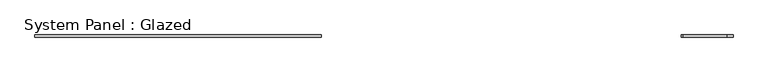
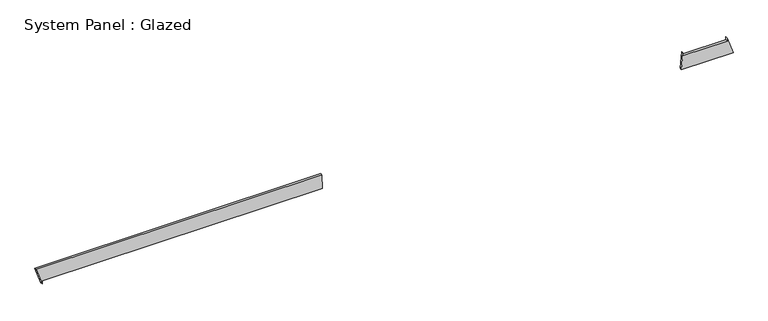
"""IFC4 building model written with IfcOpenShell, lengths in millimetres: plate geometry, System Panel : Glazed."""

import ifcopenshell
import ifcopenshell.guid

model = None  # the IFC model being written
_history = None  # IfcOwnerHistory: only IFC2X3 demands one
_inside = {}  # id of a spatial element -> (the spatial element, [elements in it])
_under = {}  # id of a project, library or spatial element -> (it, [spatial elements below it])
_declared = {}  # id of a project -> (the project, [libraries it declares])
_typed = {}  # id of a type object -> (the type object, [elements of that type])
_made_of = {}  # id of a material, layer set ... -> (it, [elements and type objects made of it])


def new_model(schema):
    """Start an empty IFC model of exactly this schema.

    Asked for "IFC4X3", IfcOpenShell would pick the latest addendum, in which some entities
    have other attributes; the version numbers below select the first issue.
    IFC2X3 requires an IfcOwnerHistory on every rooted entity: one is made here for all.
    """
    global model, _history
    if schema == "IFC4X3":
        model = ifcopenshell.file(schema_version=(4, 3, 0, 0))
    else:
        model = ifcopenshell.file(schema=schema)
    _inside.clear()
    _under.clear()
    _declared.clear()
    _typed.clear()
    _made_of.clear()
    _history = None
    if model.schema == "IFC2X3":
        org = make("IfcOrganization", Name="unknown")
        user = make(
            "IfcPersonAndOrganization",
            ThePerson=make("IfcPerson", FamilyName="unknown"),
            TheOrganization=org,
        )
        app = make(
            "IfcApplication",
            ApplicationDeveloper=org,
            Version="unknown",
            ApplicationFullName="unknown",
            ApplicationIdentifier="unknown",
        )
        _history = make(
            "IfcOwnerHistory",
            OwningUser=user,
            OwningApplication=app,
            ChangeAction="ADDED",
            CreationDate=0,
        )
    return model


def make(cls, **values):
    """One entity of the class cls with the attributes given. An attribute that is None is left unset."""
    return model.create_entity(
        cls, **{name: value for name, value in values.items() if value is not None}
    )


def rooted(cls, **values):
    """An entity with a GlobalId (a new one), such as an element, a storey or a relation."""
    return make(cls, GlobalId=ifcopenshell.guid.new(), OwnerHistory=_history, **values)


def si_unit(unit_type, name, prefix=None):
    """IfcSIUnit, for example si_unit("LENGTHUNIT", "METRE", prefix="MILLI")."""
    return make("IfcSIUnit", UnitType=unit_type, Prefix=prefix, Name=name)


def assignment(units):
    """IfcUnitAssignment: the units of a project."""
    return None if units is None else make("IfcUnitAssignment", Units=units)


def point(xyz):
    """IfcCartesianPoint."""
    return None if xyz is None else make("IfcCartesianPoint", Coordinates=xyz)


def direction(xyz):
    """IfcDirection."""
    return None if xyz is None else make("IfcDirection", DirectionRatios=xyz)


def frame(location, z_axis=None, x_axis=None):
    """IfcAxis2Placement3D, a coordinate frame: its origin and axes. An axis left out is left unset."""
    return make(
        "IfcAxis2Placement3D",
        Location=point(location),
        Axis=direction(z_axis),
        RefDirection=direction(x_axis),
    )


def origin():
    """The frame at (0, 0, 0) with its axes left unset."""
    return frame((0.0, 0.0, 0.0))


def place(relative_to, where):
    """IfcLocalPlacement: puts the frame where relative to a parent placement (None: the world)."""
    return make(
        "IfcLocalPlacement", PlacementRelTo=relative_to, RelativePlacement=where
    )


def context(
    kind, dimensions, precision=None, world=None, true_north=None, identifier=None
):
    """IfcGeometricRepresentationContext, for example the 3D "Model" context."""
    return make(
        "IfcGeometricRepresentationContext",
        ContextIdentifier=identifier,
        ContextType=kind,
        CoordinateSpaceDimension=dimensions,
        Precision=precision,
        WorldCoordinateSystem=world,
        TrueNorth=true_north,
    )


def project(units=None, contexts=None):
    """IfcProject with its units and contexts."""
    return rooted(
        "IfcProject",
        Name="project",
        RepresentationContexts=contexts,
        UnitsInContext=assignment(units),
    )


def spatial(cls, under=None, at=None, **own):
    """A site, building, storey or space (cls), placed at a placement, below another one or the project."""
    s = rooted(cls, ObjectPlacement=at, **own)
    if under is not None:
        _under.setdefault(under.id(), (under, []))[1].append(s)
    return s


def polyline(points):
    """IfcPolyline through the points."""
    return make("IfcPolyline", Points=[point(p) for p in points])


def outline(outer, holes=None, kind="AREA"):
    """IfcArbitraryClosedProfileDef: a profile drawn as a closed curve; with holes, ...WithVoids."""
    if holes is None:
        return make("IfcArbitraryClosedProfileDef", ProfileType=kind, OuterCurve=outer)
    return make(
        "IfcArbitraryProfileDefWithVoids",
        ProfileType=kind,
        OuterCurve=outer,
        InnerCurves=holes,
    )


def extrude(swept, where, along, depth):
    """IfcExtrudedAreaSolid: the profile swept, set in the frame where, extruded along a direction by depth."""
    return make(
        "IfcExtrudedAreaSolid",
        SweptArea=swept,
        Position=where,
        ExtrudedDirection=direction(along),
        Depth=depth,
    )


def shape(context_of_items, identifier, shape_type, items):
    """IfcShapeRepresentation: the items that make up one representation, for example the "Body"."""
    return make(
        "IfcShapeRepresentation",
        ContextOfItems=context_of_items,
        RepresentationIdentifier=identifier,
        RepresentationType=shape_type,
        Items=items,
    )


def source(mapping_origin, context_of_items, identifier, shape_type, items):
    """IfcRepresentationMap: a shape defined once, which mapped items show again and again."""
    return make(
        "IfcRepresentationMap",
        MappingOrigin=mapping_origin,
        MappedRepresentation=shape(context_of_items, identifier, shape_type, items),
    )


def transform(
    local_origin,
    x_axis=None,
    y_axis=None,
    z_axis=None,
    scale=None,
    scale2=None,
    scale3=None,
    uniform=True,
):
    """IfcCartesianTransformationOperator3D, or its non-uniform kind. x_axis, y_axis, z_axis: its Axis1, 2, 3."""
    if uniform:
        return make(
            "IfcCartesianTransformationOperator3D",
            Axis1=direction(x_axis),
            Axis2=direction(y_axis),
            LocalOrigin=point(local_origin),
            Scale=scale,
            Axis3=direction(z_axis),
        )
    return make(
        "IfcCartesianTransformationOperator3DnonUniform",
        Axis1=direction(x_axis),
        Axis2=direction(y_axis),
        LocalOrigin=point(local_origin),
        Scale=scale,
        Axis3=direction(z_axis),
        Scale2=scale2,
        Scale3=scale3,
    )


def mapped(mapping_source, mapping_target):
    """IfcMappedItem: shows the shape of a source again, moved by a transform."""
    return make(
        "IfcMappedItem", MappingSource=mapping_source, MappingTarget=mapping_target
    )


def made_of(thing, what):
    """Note that an element or type object is made of a material, layer set ...; save() writes the relation."""
    if what is not None:
        _made_of.setdefault(what.id(), (what, []))[1].append(thing)
    return thing


def element(
    cls,
    number,
    at=None,
    inside=None,
    cuts=None,
    type_object=None,
    material=None,
    context=None,
    identifier="Body",
    shape_type=None,
    held_by="IfcProductDefinitionShape",
    body=None,
    shapes=None,
    **own,
):
    """One element of the class cls, such as IfcWall. Its Tag is "e" and its number.

    at: its placement. inside: the storey or other place that contains it. cuts: it is an
    opening in that element (IfcRelVoidsElement). A single representation is given by context,
    identifier, shape_type and body (its items); several are given by shapes. held_by: the class
    of the entity that holds the representations. save() writes the other relations.
    """
    e = rooted(cls, Tag="e%d" % number, ObjectPlacement=at, **own)
    if body is not None:
        shapes = [shape(context, identifier, shape_type, body)]
    if shapes is not None:
        e.Representation = make(held_by, Representations=shapes)
    if inside is not None:
        _inside.setdefault(inside.id(), (inside, []))[1].append(e)
    if cuts is not None:
        rooted(
            "IfcRelVoidsElement", RelatingBuildingElement=cuts, RelatedOpeningElement=e
        )
    if type_object is not None:
        _typed.setdefault(type_object.id(), (type_object, []))[1].append(e)
    return made_of(e, material)


def aggregate(whole, parts):
    """IfcRelAggregates: a whole, such as a stair, and the parts it consists of."""
    return rooted("IfcRelAggregates", RelatingObject=whole, RelatedObjects=parts)


def save(model, path):
    """Write the relations noted so far, then the file.

    IfcRelAggregates (storeys below a building ...), IfcRelContainedInSpatialStructure (elements
    in a storey), IfcRelDefinesByType, IfcRelAssociatesMaterial and IfcRelDeclares: one each for
    every whole, place, type object, material and project.
    """
    for whole, parts in _under.values():
        aggregate(whole, parts)
    for where, things in _inside.values():
        rooted(
            "IfcRelContainedInSpatialStructure",
            RelatedElements=things,
            RelatingStructure=where,
        )
    for kind, things in _typed.values():
        rooted("IfcRelDefinesByType", RelatedObjects=things, RelatingType=kind)
    for what, things in _made_of.values():
        rooted("IfcRelAssociatesMaterial", RelatedObjects=things, RelatingMaterial=what)
    for by, libraries in _declared.values():
        rooted("IfcRelDeclares", RelatingContext=by, RelatedDefinitions=libraries)
    model.write(path)


def system_panel_glazed_58890ada(model_context):
    return source(origin(), model_context, "Body", "SweptSolid", [
        extrude(outline(polyline([(35.3553391, 3429.7598415), (35.3553391, 4028.0476561), (235.7077234, 3959.2529397), (200.3523843, 3959.2532528), (200.3478461, 3446.6577103), (235.7031851, 3446.6573973), (35.3553391, 3429.7598415)])), frame((0.0, -49.5, 0.0), z_axis=(0.0, 1.0, 0.0), x_axis=(0.0, 0.0, 1.0)), (0.0, 0.0, 1.0), 25.0),
        extrude(outline(polyline([(0.0, -3959.0814895), (35.3553391, -3959.0814895), (35.3553391, -721.6679227), (200.3109163, -724.5894165), (200.2816694, -4028.0476561), (0.0, -3959.0814895)])), frame((0.0, -49.5, 0.0), z_axis=(0.0, 1.0, 0.0), x_axis=(0.0, 0.0, 1.0)), (0.0, 0.0, 1.0), 25.0),
    ])


if __name__ == "__main__":
    model = new_model("IFC4")
    model_context = context("Model", 3, world=origin())
    ifc_project = project(units=[si_unit("LENGTHUNIT", "METRE", prefix="MILLI")], contexts=[model_context])
    site = spatial("IfcSite", under=ifc_project)
    building = spatial("IfcBuilding", under=site)
    placement = place(None, origin())
    system_panel_glazed_shape = system_panel_glazed_58890ada(model_context)
    element("IfcPlate", 1, ObjectType="System Panel : Glazed", at=placement, inside=building, context=model_context, shape_type="MappedRepresentation", body=[
        mapped(system_panel_glazed_shape, transform((0.0, 0.0, 0.0), x_axis=(1.0, 0.0, 0.0), y_axis=(0.0, 1.0, 0.0), z_axis=(0.0, 0.0, 1.0))),
    ])
    save(model, "model.ifc")

# Revit data of these elements
# Element 1 (IfcPlate, "System Panel : Glazed")
#   Materials on its faces: "Glass"
# Materials
#   "Glass": class "Glass", colour RGB 218 227 224, transparency 0.85, Description = "Soda Lime Glass", Cost = 0
